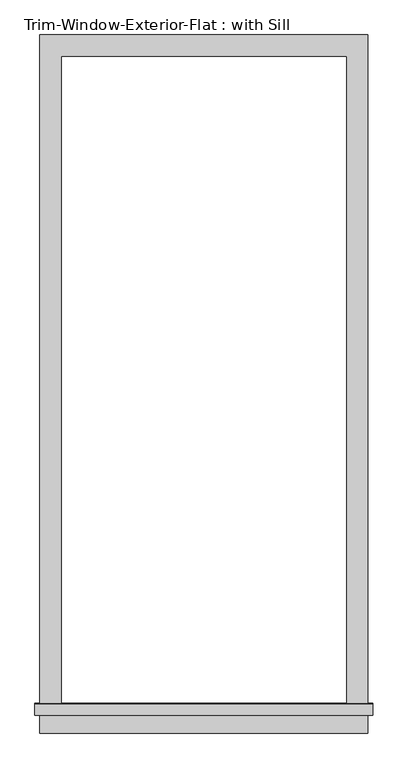
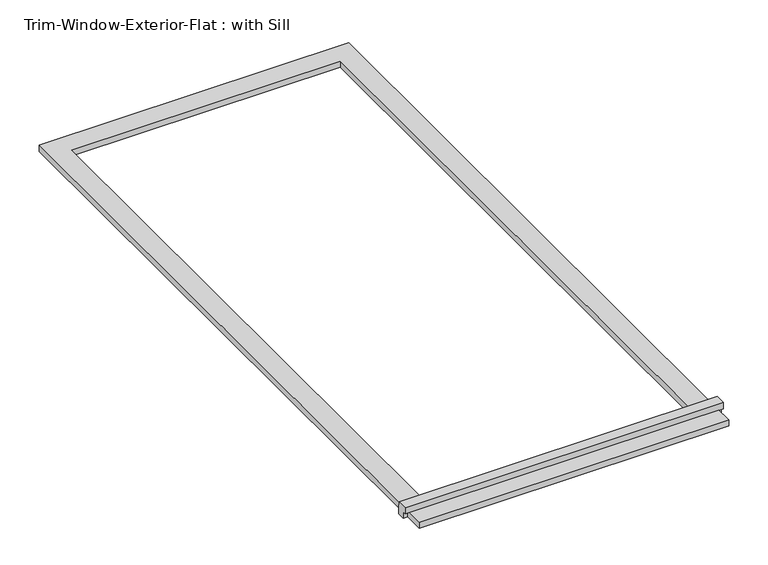
"""IFC4 building model written with IfcOpenShell, lengths in millimetres: proxy geometry, Trim-Window-Exterior-Flat : with Sill."""

from ifc_helpers import new_model, si_unit, frame, origin, origin_with_axes, place, context, project, spatial, polyline, outline, extrude, source, transform, mapped, element, save


def trim_window_exterior_flat_with_sill_b28819c4(model_context):
    return source(origin(), model_context, "Body", "SweptSolid", [
        extrude(outline(polyline([(438.15, -1749.3823709), (438.15, -1806.5323709), (-438.15, -1806.5323709), (-438.15, -1749.3823709), (438.15, -1749.3823709)])), origin_with_axes(), (0.0, 0.0, 1.0), 19.05),
        extrude(outline(polyline([(-1758.95, 38.1), (-1729.6580645, 38.1), (-1727.2, 19.05), (-1727.2, 0.0), (-1749.3823709, 0.0), (-1749.3823709, 19.05), (-1758.95, 19.05), (-1758.95, 38.1)])), frame((-450.85, 0.0, 0.0), z_axis=(1.0, 0.0, 0.0), x_axis=(0.0, 1.0, 0.0)), (0.0, 0.0, 1.0), 901.7),
        extrude(outline(polyline([(-438.15, 57.15), (438.15, 57.15), (438.15, -1727.2), (381.0, -1727.2), (381.0, 0.0), (-381.0, 0.0), (-381.0, -1727.2), (-438.15, -1727.2), (-438.15, 57.15)])), origin_with_axes(), (0.0, 0.0, 1.0), 19.05),
    ])


if __name__ == "__main__":
    model = new_model("IFC4")
    model_context = context("Model", 3, world=origin())
    ifc_project = project(units=[si_unit("LENGTHUNIT", "METRE", prefix="MILLI")], contexts=[model_context])
    site = spatial("IfcSite", under=ifc_project)
    building = spatial("IfcBuilding", under=site)
    placement = place(None, origin())
    trim_window_exterior_flat_with_sill_shape = trim_window_exterior_flat_with_sill_b28819c4(model_context)
    element("IfcBuildingElementProxy", 1, Name="Trim-Window-Exterior-Flat : with Sill", ObjectType="Trim-Window-Exterior-Flat : with Sill", at=placement, inside=building, context=model_context, shape_type="MappedRepresentation", body=[
        mapped(trim_window_exterior_flat_with_sill_shape, transform((0.0, 0.0, 0.0), x_axis=(1.0, 0.0, 0.0), y_axis=(0.0, 1.0, 0.0), z_axis=(0.0, 0.0, 1.0))),
    ])
    save(model, "model.ifc")

# Revit data of these elements
# Type "Trim-Window-Exterior-Flat : with Sill"
#   Trim Width = 0' - 2 1/4"
#   Trim Thickness_Picture Frame = 0' - 1 1/4"
#   Trim Thickness_with Sill = 0' - 0 3/4"
#   Sill Thickness = 0' - 1 1/4"
#   Opening Width [instance default] = 2' - 0"
#   Opening Height [instance default] = 3' - 0"
#   Default Elevation = 4' - 0"
#   Sill = yes
#   Picture Frame = no
#   Trim Material [instance default] = none
# Element 1 (IfcBuildingElementProxy, "Trim-Window-Exterior-Flat : with Sill")
#   Opening Width = 2' - 6"
#   Opening Height = 5' - 8"
#   Trim Material = 1X WOOD COMPOSITE TRIM
#   Materials on its faces: "1X WOOD COMPOSITE TRIM"
# Materials
#   "1X WOOD COMPOSITE TRIM": class "Generic", colour RGB 88 61 61, transparency 0, Cost = 0
